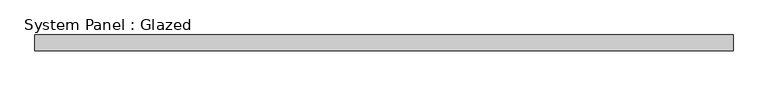
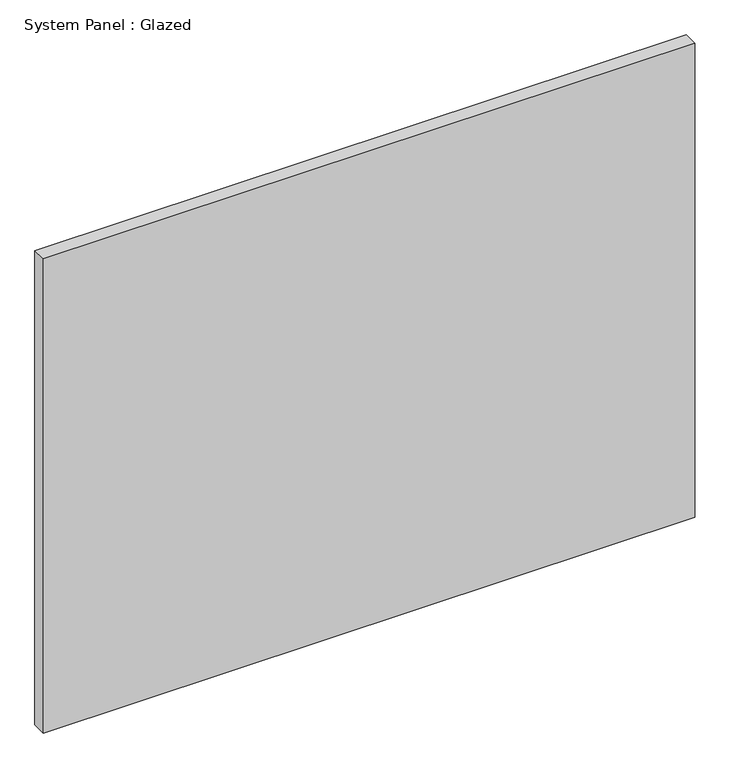
"""IFC4 building model written with IfcOpenShell, lengths in millimetres: plate geometry, System Panel : Glazed."""

import ifcopenshell
import ifcopenshell.guid

model = None  # the IFC model being written
_history = None  # IfcOwnerHistory: only IFC2X3 demands one
_inside = {}  # id of a spatial element -> (the spatial element, [elements in it])
_under = {}  # id of a project, library or spatial element -> (it, [spatial elements below it])
_declared = {}  # id of a project -> (the project, [libraries it declares])
_typed = {}  # id of a type object -> (the type object, [elements of that type])
_made_of = {}  # id of a material, layer set ... -> (it, [elements and type objects made of it])


def new_model(schema):
    """Start an empty IFC model of exactly this schema.

    Asked for "IFC4X3", IfcOpenShell would pick the latest addendum, in which some entities
    have other attributes; the version numbers below select the first issue.
    IFC2X3 requires an IfcOwnerHistory on every rooted entity: one is made here for all.
    """
    global model, _history
    if schema == "IFC4X3":
        model = ifcopenshell.file(schema_version=(4, 3, 0, 0))
    else:
        model = ifcopenshell.file(schema=schema)
    _inside.clear()
    _under.clear()
    _declared.clear()
    _typed.clear()
    _made_of.clear()
    _history = None
    if model.schema == "IFC2X3":
        org = make("IfcOrganization", Name="unknown")
        user = make(
            "IfcPersonAndOrganization",
            ThePerson=make("IfcPerson", FamilyName="unknown"),
            TheOrganization=org,
        )
        app = make(
            "IfcApplication",
            ApplicationDeveloper=org,
            Version="unknown",
            ApplicationFullName="unknown",
            ApplicationIdentifier="unknown",
        )
        _history = make(
            "IfcOwnerHistory",
            OwningUser=user,
            OwningApplication=app,
            ChangeAction="ADDED",
            CreationDate=0,
        )
    return model


def make(cls, **values):
    """One entity of the class cls with the attributes given. An attribute that is None is left unset."""
    return model.create_entity(
        cls, **{name: value for name, value in values.items() if value is not None}
    )


def rooted(cls, **values):
    """An entity with a GlobalId (a new one), such as an element, a storey or a relation."""
    return make(cls, GlobalId=ifcopenshell.guid.new(), OwnerHistory=_history, **values)


def si_unit(unit_type, name, prefix=None):
    """IfcSIUnit, for example si_unit("LENGTHUNIT", "METRE", prefix="MILLI")."""
    return make("IfcSIUnit", UnitType=unit_type, Prefix=prefix, Name=name)


def assignment(units):
    """IfcUnitAssignment: the units of a project."""
    return None if units is None else make("IfcUnitAssignment", Units=units)


def point(xyz):
    """IfcCartesianPoint."""
    return None if xyz is None else make("IfcCartesianPoint", Coordinates=xyz)


def direction(xyz):
    """IfcDirection."""
    return None if xyz is None else make("IfcDirection", DirectionRatios=xyz)


def frame(location, z_axis=None, x_axis=None):
    """IfcAxis2Placement3D, a coordinate frame: its origin and axes. An axis left out is left unset."""
    return make(
        "IfcAxis2Placement3D",
        Location=point(location),
        Axis=direction(z_axis),
        RefDirection=direction(x_axis),
    )


def origin():
    """The frame at (0, 0, 0) with its axes left unset."""
    return frame((0.0, 0.0, 0.0))


def origin_with_axes():
    """The frame at (0, 0, 0) with the z axis (0, 0, 1) and the x axis (1, 0, 0) written out."""
    return frame((0.0, 0.0, 0.0), z_axis=(0.0, 0.0, 1.0), x_axis=(1.0, 0.0, 0.0))


def place(relative_to, where):
    """IfcLocalPlacement: puts the frame where relative to a parent placement (None: the world)."""
    return make(
        "IfcLocalPlacement", PlacementRelTo=relative_to, RelativePlacement=where
    )


def context(
    kind, dimensions, precision=None, world=None, true_north=None, identifier=None
):
    """IfcGeometricRepresentationContext, for example the 3D "Model" context."""
    return make(
        "IfcGeometricRepresentationContext",
        ContextIdentifier=identifier,
        ContextType=kind,
        CoordinateSpaceDimension=dimensions,
        Precision=precision,
        WorldCoordinateSystem=world,
        TrueNorth=true_north,
    )


def project(units=None, contexts=None):
    """IfcProject with its units and contexts."""
    return rooted(
        "IfcProject",
        Name="project",
        RepresentationContexts=contexts,
        UnitsInContext=assignment(units),
    )


def spatial(cls, under=None, at=None, **own):
    """A site, building, storey or space (cls), placed at a placement, below another one or the project."""
    s = rooted(cls, ObjectPlacement=at, **own)
    if under is not None:
        _under.setdefault(under.id(), (under, []))[1].append(s)
    return s


def polyline(points):
    """IfcPolyline through the points."""
    return make("IfcPolyline", Points=[point(p) for p in points])


def outline(outer, holes=None, kind="AREA"):
    """IfcArbitraryClosedProfileDef: a profile drawn as a closed curve; with holes, ...WithVoids."""
    if holes is None:
        return make("IfcArbitraryClosedProfileDef", ProfileType=kind, OuterCurve=outer)
    return make(
        "IfcArbitraryProfileDefWithVoids",
        ProfileType=kind,
        OuterCurve=outer,
        InnerCurves=holes,
    )


def extrude(swept, where, along, depth):
    """IfcExtrudedAreaSolid: the profile swept, set in the frame where, extruded along a direction by depth."""
    return make(
        "IfcExtrudedAreaSolid",
        SweptArea=swept,
        Position=where,
        ExtrudedDirection=direction(along),
        Depth=depth,
    )


def shape(context_of_items, identifier, shape_type, items):
    """IfcShapeRepresentation: the items that make up one representation, for example the "Body"."""
    return make(
        "IfcShapeRepresentation",
        ContextOfItems=context_of_items,
        RepresentationIdentifier=identifier,
        RepresentationType=shape_type,
        Items=items,
    )


def source(mapping_origin, context_of_items, identifier, shape_type, items):
    """IfcRepresentationMap: a shape defined once, which mapped items show again and again."""
    return make(
        "IfcRepresentationMap",
        MappingOrigin=mapping_origin,
        MappedRepresentation=shape(context_of_items, identifier, shape_type, items),
    )


def transform(
    local_origin,
    x_axis=None,
    y_axis=None,
    z_axis=None,
    scale=None,
    scale2=None,
    scale3=None,
    uniform=True,
):
    """IfcCartesianTransformationOperator3D, or its non-uniform kind. x_axis, y_axis, z_axis: its Axis1, 2, 3."""
    if uniform:
        return make(
            "IfcCartesianTransformationOperator3D",
            Axis1=direction(x_axis),
            Axis2=direction(y_axis),
            LocalOrigin=point(local_origin),
            Scale=scale,
            Axis3=direction(z_axis),
        )
    return make(
        "IfcCartesianTransformationOperator3DnonUniform",
        Axis1=direction(x_axis),
        Axis2=direction(y_axis),
        LocalOrigin=point(local_origin),
        Scale=scale,
        Axis3=direction(z_axis),
        Scale2=scale2,
        Scale3=scale3,
    )


def mapped(mapping_source, mapping_target):
    """IfcMappedItem: shows the shape of a source again, moved by a transform."""
    return make(
        "IfcMappedItem", MappingSource=mapping_source, MappingTarget=mapping_target
    )


def made_of(thing, what):
    """Note that an element or type object is made of a material, layer set ...; save() writes the relation."""
    if what is not None:
        _made_of.setdefault(what.id(), (what, []))[1].append(thing)
    return thing


def element(
    cls,
    number,
    at=None,
    inside=None,
    cuts=None,
    type_object=None,
    material=None,
    context=None,
    identifier="Body",
    shape_type=None,
    held_by="IfcProductDefinitionShape",
    body=None,
    shapes=None,
    **own,
):
    """One element of the class cls, such as IfcWall. Its Tag is "e" and its number.

    at: its placement. inside: the storey or other place that contains it. cuts: it is an
    opening in that element (IfcRelVoidsElement). A single representation is given by context,
    identifier, shape_type and body (its items); several are given by shapes. held_by: the class
    of the entity that holds the representations. save() writes the other relations.
    """
    e = rooted(cls, Tag="e%d" % number, ObjectPlacement=at, **own)
    if body is not None:
        shapes = [shape(context, identifier, shape_type, body)]
    if shapes is not None:
        e.Representation = make(held_by, Representations=shapes)
    if inside is not None:
        _inside.setdefault(inside.id(), (inside, []))[1].append(e)
    if cuts is not None:
        rooted(
            "IfcRelVoidsElement", RelatingBuildingElement=cuts, RelatedOpeningElement=e
        )
    if type_object is not None:
        _typed.setdefault(type_object.id(), (type_object, []))[1].append(e)
    return made_of(e, material)


def aggregate(whole, parts):
    """IfcRelAggregates: a whole, such as a stair, and the parts it consists of."""
    return rooted("IfcRelAggregates", RelatingObject=whole, RelatedObjects=parts)


def save(model, path):
    """Write the relations noted so far, then the file.

    IfcRelAggregates (storeys below a building ...), IfcRelContainedInSpatialStructure (elements
    in a storey), IfcRelDefinesByType, IfcRelAssociatesMaterial and IfcRelDeclares: one each for
    every whole, place, type object, material and project.
    """
    for whole, parts in _under.values():
        aggregate(whole, parts)
    for where, things in _inside.values():
        rooted(
            "IfcRelContainedInSpatialStructure",
            RelatedElements=things,
            RelatingStructure=where,
        )
    for kind, things in _typed.values():
        rooted("IfcRelDefinesByType", RelatedObjects=things, RelatingType=kind)
    for what, things in _made_of.values():
        rooted("IfcRelAssociatesMaterial", RelatedObjects=things, RelatingMaterial=what)
    for by, libraries in _declared.values():
        rooted("IfcRelDeclares", RelatingContext=by, RelatedDefinitions=libraries)
    model.write(path)


def system_panel_glazed_087d2106(model_context):
    return source(origin(), model_context, "Body", "SweptSolid", [
        extrude(outline(polyline([(565.15, 19.05), (-565.15, 19.05), (-565.15, 44.45), (565.15, 44.45), (565.15, 19.05)])), origin_with_axes(), (0.0, 0.0, 1.0), 869.95),
    ])


if __name__ == "__main__":
    model = new_model("IFC4")
    model_context = context("Model", 3, world=origin())
    ifc_project = project(units=[si_unit("LENGTHUNIT", "METRE", prefix="MILLI")], contexts=[model_context])
    site = spatial("IfcSite", under=ifc_project)
    building = spatial("IfcBuilding", under=site)
    placement = place(None, origin())
    system_panel_glazed_shape = system_panel_glazed_087d2106(model_context)
    element("IfcPlate", 1, ObjectType="System Panel : Glazed", at=placement, inside=building, context=model_context, shape_type="MappedRepresentation", body=[
        mapped(system_panel_glazed_shape, transform((0.0, 0.0, 0.0), x_axis=(1.0, 0.0, 0.0), y_axis=(0.0, 1.0, 0.0), z_axis=(0.0, 0.0, 1.0))),
    ])
    save(model, "model.ifc")

# Revit data of these elements
# Element 1 (IfcPlate, "System Panel : Glazed")
#   Materials on its faces: "Glass"
# Materials
#   "Glass": class "Glass", colour RGB 0 128 192, transparency 0.75
